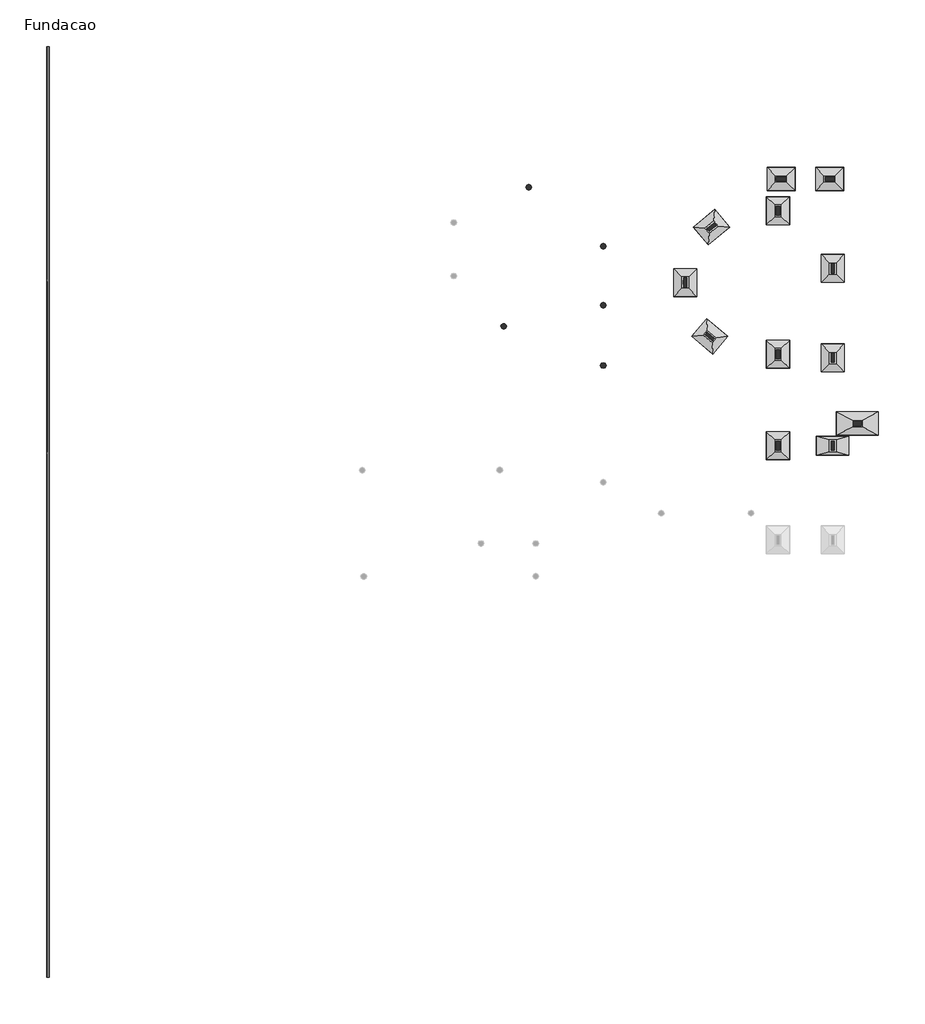
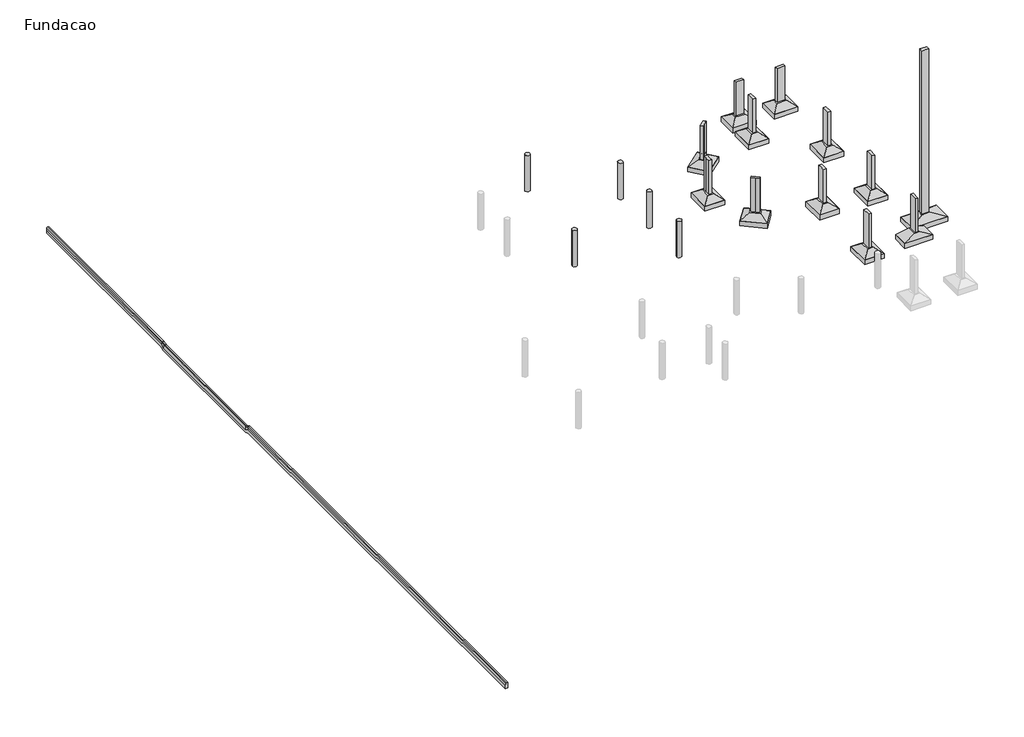
# One storey, part 2 of 2: 17 columns, 12 fasteners, 1 proxy.
# Revit data of these elements (continued)
# Element 4 (IfcColumn, "TQS - Pilar circular : TQS - Pilar circular 25.0cm") (continued)
#   Unir com o próximo = ""
#   Grupo pre moldado = ""
#   Verificado = ""
#   Concreto C = ""
#   Taxa de armadura (kgf/m³) = 0
#   Carga (tf/m²) = 0
#   Carga (tf/m) = 0
#   Carga (tf) = 0
#   Altura = 1.70 m
#   Rebaixo = 0.00 m
#   Altura da fundacao = 0.00 m
#   Largura = 0.00 m
#   Distancia a face = 0.00 m
#   Distancia ao eixo = 0.00 m
#   Resultado de Ensaios fck (MPa) = 0
#   Unique TQS ID = -767
#   Principal = yes
#   Nasce = yes
#   Morre = yes
#   Cabeca de Pilar = no
#   Structural Material = Concrete - Cast-in-Place Concrete
#   Phase Created = CC_AP/ESTR
#   Materials on its faces: "Concrete - Cast-in-Place Concrete"
# Element 5 (IfcColumn, "TQS - Pilar circular : TQS - Pilar circular 25.0cm")
#   Uso = "ESTRUTURA"
#   Titulo = "B3"
#   Chave = "B3//0"
#   Tipo Elemento = "Pilar"
#   SHA1 = "B4824BA6EB04DBA88013BAD919A11F987E93A8CE"
#   Revisão = ""
#   Tipo de carga = ""
#   Divisor de flexao = ""
#   Secao = "C 25"
#   Configuracao = ""
#   Angulo (graus) = ""
#   Detalhamento = ""
#   Casos de vento manual = ""
#   Tipo = ""
#   Alcas = ""
#   Furos = ""
#   Pino = ""
#   Distribuicao = ""
#   Solidarizado = ""
#   Solidarizar na montagem = ""
#   Unir com o próximo = ""
#   Grupo pre moldado = ""
#   Verificado = ""
#   Concreto C = ""
#   Taxa de armadura (kgf/m³) = 0
#   Carga (tf/m²) = 0
#   Carga (tf/m) = 0
#   Carga (tf) = 0
#   Altura = 1.70 m
#   Rebaixo = 0.00 m
#   Altura da fundacao = 0.00 m
#   Largura = 0.00 m
#   Distancia a face = 0.00 m
#   Distancia ao eixo = 0.00 m
#   Resultado de Ensaios fck (MPa) = 0
#   Unique TQS ID = -768
#   Principal = yes
#   Nasce = yes
#   Morre = yes
#   Cabeca de Pilar = no
#   Structural Material = Concrete - Cast-in-Place Concrete
#   Phase Created = CC_AP/ESTR
#   Materials on its faces: "Concrete - Cast-in-Place Concrete"
# Element 6 (IfcColumn, "TQS - Pilar circular : TQS - Pilar circular 25.0cm")
#   Uso = "ESTRUTURA"
#   Titulo = "B7"
#   Chave = "B7//0"
#   Tipo Elemento = "Pilar"
#   SHA1 = "0C09F8E52B5679DF636ED6AD079635606BCF1DE0"
#   Revisão = ""
#   Tipo de carga = ""
#   Divisor de flexao = ""
#   Secao = "C 25"
#   Configuracao = ""
#   Angulo (graus) = ""
#   Detalhamento = ""
#   Casos de vento manual = ""
#   Tipo = ""
#   Alcas = ""
#   Furos = ""
#   Pino = ""
#   Distribuicao = ""
#   Solidarizado = ""
#   Solidarizar na montagem = ""
#   Unir com o próximo = ""
#   Grupo pre moldado = ""
#   Verificado = ""
#   Concreto C = ""
#   Taxa de armadura (kgf/m³) = 0
#   Carga (tf/m²) = 0
#   Carga (tf/m) = 0
#   Carga (tf) = 0
#   Altura = 1.70 m
#   Rebaixo = 0.00 m
#   Altura da fundacao = 0.00 m
#   Largura = 0.00 m
#   Distancia a face = 0.00 m
#   Distancia ao eixo = 0.00 m
#   Resultado de Ensaios fck (MPa) = 0
#   Unique TQS ID = -769
#   Principal = yes
#   Nasce = yes
#   Morre = yes
#   Cabeca de Pilar = no
#   Structural Material = Concrete - Cast-in-Place Concrete
#   Phase Created = CC_AP/ESTR
#   Materials on its faces: "Concrete - Cast-in-Place Concrete"
# Element 7 (IfcColumn, "TQS - Pilar retangular : 14.0 x 40.0")
#   Uso = "ESTRUTURA"
#   Titulo = "PS1"
#   Chave = "PS1//0"
#   Tipo Elemento = "Pilar"
#   SHA1 = "4597F8CE5B5008DD3216867DEF2D1334C590FC15"
#   Revisão = ""
#   Tipo de carga = ""
#   Divisor de flexao = ""
#   Secao = "R 14/40 270°"
#   Configuracao = ""
#   Angulo (graus) = ""
#   Detalhamento = ""
#   Casos de vento manual = ""
#   Tipo = ""
#   Alcas = ""
#   Furos = ""
#   Pino = ""
#   Distribuicao = ""
#   Solidarizado = ""
#   Solidarizar na montagem = ""
#   Unir com o próximo = ""
#   Grupo pre moldado = ""
#   Verificado = ""
#   Concreto C = ""
#   Taxa de armadura (kgf/m³) = 0
#   Carga (tf/m²) = 0
#   Carga (tf/m) = 0
#   Carga (tf) = 0
#   Altura = 1.70 m
#   Rebaixo = 0.00 m
#   Altura da fundacao = 0.00 m
#   Largura = 0.00 m
#   Distancia a face = 0.00 m
#   Distancia ao eixo = 0.00 m
#   Resultado de Ensaios fck (MPa) = 0
#   Unique TQS ID = -958
#   Principal = yes
#   Nasce = yes
#   Morre = yes
#   Cabeca de Pilar = no
#   Structural Material = Concrete - Cast-in-Place Concrete
#   Phase Created = CC_AP/ESTR
#   Materials on its faces: "Concrete - Cast-in-Place Concrete"
# Element 8 (IfcColumn, "TQS - Pilar retangular : 14.0 x 40.0")
#   Uso = "ESTRUTURA"
#   Titulo = "PS2"
#   Chave = "PS2//0"
#   Tipo Elemento = "Pilar"
#   SHA1 = "1729CD9DA72122FACD843418D908847D3B1966CD"
#   Revisão = ""
#   Tipo de carga = ""
#   Divisor de flexao = ""
#   Secao = "R 14/40 270°"
#   Configuracao = ""
#   Angulo (graus) = ""
#   Detalhamento = ""
#   Casos de vento manual = ""
#   Tipo = ""
#   Alcas = ""
#   Furos = ""
#   Pino = ""
#   Distribuicao = ""
#   Solidarizado = ""
#   Solidarizar na montagem = ""
#   Unir com o próximo = ""
#   Grupo pre moldado = ""
#   Verificado = ""
#   Concreto C = ""
#   Taxa de armadura (kgf/m³) = 0
#   Carga (tf/m²) = 0
#   Carga (tf/m) = 0
#   Carga (tf) = 0
#   Altura = 1.70 m
#   Rebaixo = 0.00 m
#   Altura da fundacao = 0.00 m
#   Largura = 0.00 m
#   Distancia a face = 0.00 m
#   Distancia ao eixo = 0.00 m
#   Resultado de Ensaios fck (MPa) = 0
#   Unique TQS ID = -959
#   Principal = yes
#   Nasce = yes
#   Morre = yes
#   Cabeca de Pilar = no
#   Structural Material = Concrete - Cast-in-Place Concrete
#   Phase Created = CC_AP/ESTR
#   Materials on its faces: "Concrete - Cast-in-Place Concrete"
# Element 9 (IfcColumn, "TQS - Pilar retangular : 14.0 x 40.0")
#   Uso = "ESTRUTURA"
#   Titulo = "PS3"
#   Chave = "PS3//0"
#   Tipo Elemento = "Pilar"
#   SHA1 = "E1C4E1DD2B85E2F78CE9D8770BC24705A0EC4463"
#   Revisão = ""
#   Tipo de carga = ""
#   Divisor de flexao = ""
#   Secao = "R 14/40 180°"
#   Configuracao = ""
#   Angulo (graus) = ""
#   Detalhamento = ""
#   Casos de vento manual = ""
#   Tipo = ""
#   Alcas = ""
#   Furos = ""
#   Pino = ""
#   Distribuicao = ""
#   Solidarizado = ""
#   Solidarizar na montagem = ""
#   Unir com o próximo = ""
#   Grupo pre moldado = ""
#   Verificado = ""
#   Concreto C = ""
#   Taxa de armadura (kgf/m³) = 0
#   Carga (tf/m²) = 0
#   Carga (tf/m) = 0
#   Carga (tf) = 0
#   Altura = 1.70 m
#   Rebaixo = 0.00 m
#   Altura da fundacao = 0.00 m
#   Largura = 0.00 m
#   Distancia a face = 0.00 m
#   Distancia ao eixo = 0.00 m
#   Resultado de Ensaios fck (MPa) = 0
#   Unique TQS ID = -960
#   Principal = yes
#   Nasce = yes
#   Morre = yes
#   Cabeca de Pilar = no
#   Structural Material = Concrete - Cast-in-Place Concrete
#   Phase Created = CC_AP/ESTR
#   Materials on its faces: "Concrete - Cast-in-Place Concrete"
# Element 10 (IfcColumn, "TQS - Pilar retangular : 14.0 x 40.0")
#   Uso = "ESTRUTURA"
#   Titulo = "PS7"
#   Chave = "PS7//0"
#   Tipo Elemento = "Pilar"
#   SHA1 = "EE51B7F018C373FE9CEF53A9864C8051348A9FB9"
#   Revisão = ""
#   Tipo de carga = ""
#   Divisor de flexao = ""
#   Secao = "R 14/40 180°"
#   Configuracao = ""
#   Angulo (graus) = ""
#   Detalhamento = ""
#   Casos de vento manual = ""
#   Tipo = ""
#   Alcas = ""
#   Furos = ""
#   Pino = ""
#   Distribuicao = ""
#   Solidarizado = ""
#   Solidarizar na montagem = ""
#   Unir com o próximo = ""
#   Grupo pre moldado = ""
#   Verificado = ""
#   Concreto C = ""
#   Taxa de armadura (kgf/m³) = 0
#   Carga (tf/m²) = 0
#   Carga (tf/m) = 0
#   Carga (tf) = 0
#   Altura = 1.70 m
#   Rebaixo = 0.00 m
#   Altura da fundacao = 0.00 m
#   Largura = 0.00 m
#   Distancia a face = 0.00 m
#   Distancia ao eixo = 0.00 m
#   Resultado de Ensaios fck (MPa) = 0
#   Unique TQS ID = -964
#   Principal = yes
#   Nasce = yes
#   Morre = yes
#   Cabeca de Pilar = no
#   Structural Material = Concrete - Cast-in-Place Concrete
#   Phase Created = CC_AP/ESTR
#   Materials on its faces: "Concrete - Cast-in-Place Concrete"
# Element 11 (IfcColumn, "TQS - Pilar retangular : 14.0 x 40.0")
#   Uso = "ESTRUTURA"
#   Titulo = "PS8"
#   Chave = "PS8//0"
#   Tipo Elemento = "Pilar"
#   SHA1 = "B515A8CC25CBD0A114828B82A1075E16319BC015"
#   Revisão = ""
#   Tipo de carga = ""
#   Divisor de flexao = ""
#   Secao = "R 14/40 180°"
#   Configuracao = ""
#   Angulo (graus) = ""
#   Detalhamento = ""
#   Casos de vento manual = ""
#   Tipo = ""
#   Alcas = ""
#   Furos = ""
#   Pino = ""
#   Distribuicao = ""
#   Solidarizado = ""
#   Solidarizar na montagem = ""
#   Unir com o próximo = ""
#   Grupo pre moldado = ""
#   Verificado = ""
#   Concreto C = ""
#   Taxa de armadura (kgf/m³) = 0
#   Carga (tf/m²) = 0
#   Carga (tf/m) = 0
#   Carga (tf) = 0
#   Altura = 1.70 m
#   Rebaixo = 0.00 m
#   Altura da fundacao = 0.00 m
#   Largura = 0.00 m
#   Distancia a face = 0.00 m
#   Distancia ao eixo = 0.00 m
#   Resultado de Ensaios fck (MPa) = 0
#   Unique TQS ID = -965
#   Principal = yes
#   Nasce = yes
#   Morre = yes
#   Cabeca de Pilar = no
#   Structural Material = Concrete - Cast-in-Place Concrete
#   Phase Created = CC_AP/ESTR
#   Materials on its faces: "Concrete - Cast-in-Place Concrete"
# Element 12 (IfcColumn, "TQS - Pilar retangular : 14.0 x 40.0")
#   Uso = "ESTRUTURA"
#   Titulo = "PS11"
#   Chave = "PS11//0"
#   Tipo Elemento = "Pilar"
#   SHA1 = "38C3E9E25C80C043D595FE86FE1A911FDC38D350"
#   Revisão = ""
#   Tipo de carga = ""
#   Divisor de flexao = ""
#   Secao = "R 14/40 180°"
#   Configuracao = ""
#   Angulo (graus) = ""
#   Detalhamento = ""
#   Casos de vento manual = ""
#   Tipo = ""
#   Alcas = ""
#   Furos = ""
#   Pino = ""
#   Distribuicao = ""
#   Solidarizado = ""
#   Solidarizar na montagem = ""
#   Unir com o próximo = ""
#   Grupo pre moldado = ""
#   Verificado = ""
#   Concreto C = ""
#   Taxa de armadura (kgf/m³) = 0
#   Carga (tf/m²) = 0
#   Carga (tf/m) = 0
#   Carga (tf) = 0
#   Altura = 1.70 m
#   Rebaixo = 0.00 m
#   Altura da fundacao = 0.00 m
#   Largura = 0.00 m
#   Distancia a face = 0.00 m
#   Distancia ao eixo = 0.00 m
#   Resultado de Ensaios fck (MPa) = 0
#   Unique TQS ID = -968
#   Principal = yes
#   Nasce = yes
#   Morre = yes
#   Cabeca de Pilar = no
#   Structural Material = Concrete - Cast-in-Place Concrete
#   Phase Created = CC_AP/ESTR
#   Materials on its faces: "Concrete - Cast-in-Place Concrete"
# Element 13 (IfcColumn, "TQS - Pilar retangular : 14.0 x 40.0")
#   Uso = "ESTRUTURA"
#   Titulo = "PS12"
#   Chave = "PS12//0"
#   Tipo Elemento = "Pilar"
#   SHA1 = "512D0DE7DB718BC0FE0AECE12A9FB23F7FBE26A9"
#   Revisão = ""
#   Tipo de carga = ""
#   Divisor de flexao = ""
#   Secao = "R 14/40 180°"
#   Configuracao = ""
#   Angulo (graus) = ""
#   Detalhamento = ""
#   Casos de vento manual = ""
#   Tipo = ""
#   Alcas = ""
#   Furos = ""
#   Pino = ""
#   Distribuicao = ""
#   Solidarizado = ""
#   Solidarizar na montagem = ""
#   Unir com o próximo = ""
#   Grupo pre moldado = ""
#   Verificado = ""
#   Concreto C = ""
#   Taxa de armadura (kgf/m³) = 0
#   Carga (tf/m²) = 0
#   Carga (tf/m) = 0
#   Carga (tf) = 0
#   Altura = 1.70 m
#   Rebaixo = 0.00 m
#   Altura da fundacao = 0.00 m
#   Largura = 0.00 m
#   Distancia a face = 0.00 m
#   Distancia ao eixo = 0.00 m
#   Resultado de Ensaios fck (MPa) = 0
#   Unique TQS ID = -969
#   Principal = yes
#   Nasce = yes
#   Morre = yes
#   Cabeca de Pilar = no
#   Structural Material = Concrete - Cast-in-Place Concrete
#   Phase Created = CC_AP/ESTR
#   Materials on its faces: "Concrete - Cast-in-Place Concrete"
# Element 14 (IfcColumn, "TQS - Pilar retangular : 14.0 x 40.0")
#   Uso = "ESTRUTURA"
#   Titulo = "PS13"
#   Chave = "PS13//0"
#   Tipo Elemento = "Pilar"
#   SHA1 = "8EC8E2C6B90DD4DF760F1D4ED431316ED84D10F2"
#   Revisão = ""
#   Tipo de carga = ""
#   Divisor de flexao = ""
#   Secao = "R 14/40 180°"
#   Configuracao = ""
#   Angulo (graus) = ""
#   Detalhamento = ""
#   Casos de vento manual = ""
#   Tipo = ""
#   Alcas = ""
#   Furos = ""
#   Pino = ""
#   Distribuicao = ""
#   Solidarizado = ""
#   Solidarizar na montagem = ""
#   Unir com o próximo = ""
#   Grupo pre moldado = ""
#   Verificado = ""
#   Concreto C = ""
#   Taxa de armadura (kgf/m³) = 0
#   Carga (tf/m²) = 0
#   Carga (tf/m) = 0
#   Carga (tf) = 0
#   Altura = 1.70 m
#   Rebaixo = 0.00 m
#   Altura da fundacao = 0.00 m
#   Largura = 0.00 m
#   Distancia a face = 0.00 m
#   Distancia ao eixo = 0.00 m
#   Resultado de Ensaios fck (MPa) = 0
#   Unique TQS ID = -970
#   Principal = yes
#   Nasce = yes
#   Morre = yes
#   Cabeca de Pilar = no
#   Structural Material = Concrete - Cast-in-Place Concrete
#   Phase Created = CC_AP/ESTR
#   Materials on its faces: "Concrete - Cast-in-Place Concrete"
# Element 15 (IfcColumn, "TQS - Pilar retangular : 19.0 x 35.0")
#   Uso = "ESTRUTURA"
#   Titulo = "P14"
#   Chave = "P14//0"
#   Tipo Elemento = "Pilar"
#   SHA1 = "6631C03D899D7914EBA5EACF44BE1498A45C603B"
#   Revisão = ""
#   Tipo de carga = ""
#   Divisor de flexao = ""
#   Secao = "R 19/35 90°"
#   Configuracao = ""
#   Angulo (graus) = ""
#   Detalhamento = ""
#   Casos de vento manual = ""
#   Tipo = ""
#   Alcas = ""
#   Furos = ""
#   Pino = ""
#   Distribuicao = ""
#   Solidarizado = ""
#   Solidarizar na montagem = ""
#   Unir com o próximo = ""
#   Grupo pre moldado = ""
#   Verificado = ""
#   Concreto C = ""
#   Taxa de armadura (kgf/m³) = 0
#   Carga (tf/m²) = 0
#   Carga (tf/m) = 0
#   Carga (tf) = 0
#   Altura = 7.85 m
#   Rebaixo = 0.00 m
#   Altura da fundacao = 0.00 m
#   Largura = 0.00 m
#   Distancia a face = 0.00 m
#   Distancia ao eixo = 0.00 m
#   Resultado de Ensaios fck (MPa) = 0
#   Unique TQS ID = -30
#   Principal = yes
#   Nasce = yes
#   Morre = yes
#   Cabeca de Pilar = no
#   Structural Material = Concrete - Cast-in-Place Concrete
#   Phase Created = CC_AP/ESTR
#   Materials on its faces: "Concrete - Cast-in-Place Concrete"
# Element 16 (IfcColumn, "TQS - Pilar Polig_1 : TQS Column")
#   Uso = "ESTRUTURA"
#   Titulo = "PS4"
#   Chave = "PS4//0"
#   Tipo Elemento = "Pilar"
#   SHA1 = "CAF5758E71A5FE097847EBD6542E0EE23CE53B7B"
#   Revisão = ""
#   Tipo de carga = ""
#   Divisor de flexao = ""
#   Secao = "P  - Poligonal"
#   Configuracao = ""
#   Angulo (graus) = ""
#   Detalhamento = ""
#   Casos de vento manual = ""
#   Tipo = ""
#   Alcas = ""
#   Furos = ""
#   Pino = ""
#   Distribuicao = ""
#   Solidarizado = ""
#   Solidarizar na montagem = ""
#   Unir com o próximo = ""
#   Grupo pre moldado = ""
#   Verificado = ""
#   Concreto C = ""
#   Taxa de armadura (kgf/m³) = 0
#   Carga (tf/m²) = 0
#   Carga (tf/m) = 0
#   Carga (tf) = 0
#   Altura = 1.70 m
#   Rebaixo = 0.00 m
#   Altura da fundacao = 0.00 m
#   Largura = 0.00 m
#   Distancia a face = 0.00 m
#   Distancia ao eixo = 0.00 m
#   Resultado de Ensaios fck (MPa) = 0
#   Unique TQS ID = -961
#   Principal = yes
#   Nasce = yes
#   Morre = yes
#   Cabeca de Pilar = no
#   Structural Material = Concrete - Cast-in-Place Concrete
#   Phase Created = CC_AP/ESTR
# Element 17 (IfcColumn, "TQS - Pilar Polig_1 : TQS Column")
#   Uso = "ESTRUTURA"
#   Titulo = "PS5"
#   Chave = "PS5//0"
#   Tipo Elemento = "Pilar"
#   SHA1 = "AE9BDBDC0B1786B9555B7E0CE4AAD4E849800AD1"
#   Revisão = ""
#   Tipo de carga = ""
#   Divisor de flexao = ""
#   Secao = "P  - Poligonal"
#   Configuracao = ""
#   Angulo (graus) = ""
#   Detalhamento = ""
#   Casos de vento manual = ""
#   Tipo = ""
#   Alcas = ""
#   Furos = ""
#   Pino = ""
#   Distribuicao = ""
#   Solidarizado = ""
#   Solidarizar na montagem = ""
#   Unir com o próximo = ""
#   Grupo pre moldado = ""
#   Verificado = ""
#   Concreto C = ""
#   Taxa de armadura (kgf/m³) = 0
#   Carga (tf/m²) = 0
#   Carga (tf/m) = 0
#   Carga (tf) = 0
#   Altura = 1.70 m
#   Rebaixo = 0.00 m
#   Altura da fundacao = 0.00 m
#   Largura = 0.00 m
#   Distancia a face = 0.00 m
#   Distancia ao eixo = 0.00 m
#   Resultado de Ensaios fck (MPa) = 0
#   Unique TQS ID = -962
#   Principal = yes
#   Nasce = yes
#   Morre = yes
#   Cabeca de Pilar = no
#   Structural Material = Concrete - Cast-in-Place Concrete
#   Phase Created = CC_AP/ESTR
# Element 18 (IfcColumn, "TQS - Pilar Polig_2 : TQS Column")
#   Uso = "ESTRUTURA"
#   Titulo = "PS6"
#   Chave = "PS6//0"
#   Tipo Elemento = "Pilar"
#   SHA1 = "07EEAEB0E5A3D9C7C5812BCB6FDA506A68E4D4F2"
#   Revisão = ""
#   Tipo de carga = ""
#   Divisor de flexao = ""
#   Secao = "P  - Poligonal"
#   Configuracao = ""
#   Angulo (graus) = ""
#   Detalhamento = ""
#   Casos de vento manual = ""
#   Tipo = ""
#   Alcas = ""
#   Furos = ""
#   Pino = ""
#   Distribuicao = ""
#   Solidarizado = ""
#   Solidarizar na montagem = ""
#   Unir com o próximo = ""
#   Grupo pre moldado = ""
#   Verificado = ""
#   Concreto C = ""
#   Taxa de armadura (kgf/m³) = 0
#   Carga (tf/m²) = 0
#   Carga (tf/m) = 0
#   Carga (tf) = 0
#   Altura = 1.70 m
#   Rebaixo = 0.00 m
#   Altura da fundacao = 0.00 m
#   Largura = 0.00 m
#   Distancia a face = 0.00 m
#   Distancia ao eixo = 0.00 m
#   Resultado de Ensaios fck (MPa) = 0
#   Unique TQS ID = -963
#   Principal = yes
#   Nasce = yes
#   Morre = yes
#   Cabeca de Pilar = no
#   Structural Material = Concrete - Cast-in-Place Concrete
#   Phase Created = CC_AP/ESTR
# Element 19 (IfcFastener, "TQS - Sapata : S14")
#   Uso = "ESTRUTURA"
#   Titulo = "S14"
#   Chave = "-1550"
#   Tipo Elemento = "Fundação"
#   SHA1 = "1357E856F80250D7EFC9EC1E050D5963CC884844"
#   Revisão = ""
#   Tipo de carga = ""
#   Divisor de flexao = ""
#   Secao = ""
#   Configuracao = ""
#   Angulo (graus) = ""
#   Detalhamento = ""
#   Casos de vento manual = ""
#   Tipo = "Sapata"
#   Dimensoes = "100.0,180.0"
#   Estacas = ""
#   Calice = ""
#   Rugosidade = ""
#   Alcas = ""
#   Furos = ""
#   Pino = ""
#   Distribuicao = ""
#   Solidarizado = ""
#   Solidarizar na montagem = ""
#   Unir com o próximo = ""
#   Grupo pre moldado = ""
#   Verificado = ""
#   Concreto C = ""
#   Taxa de armadura (kgf/m³) = 0
#   Carga (tf/m²) = 0
#   Carga (tf/m) = 0
#   Carga (tf) = 0
#   Altura = 0.00 m
#   Rebaixo = 0.00 m
#   Pilar ficticio = 0.00 m
#   Topo = -1.45 m
#   Altura total = 0.50 m
#   Rodape = 0.00 m
#   Diametro = 0.00 m
#   Altura dentro do bloco = 0.00 m
#   Entre eixos = 0.00 m
#   Paredes = 0.00 m
#   Caimento = 0.00 m
#   Largura = 0.00 m
#   Distancia a face = 0.00 m
#   Distancia ao eixo = 0.00 m
#   Resultado de Ensaios fck (MPa) = 0
#   Unique TQS ID = -1550
#   Principal = yes
#   Phase Created = CC_AP/ESTR
#   Materials on its faces: "Concreto - Concreto concretado no local"
# Element 20 (IfcFastener, "TQS - Sapata : SPS1")
#   Uso = "ESTRUTURA"
#   Titulo = "SPS1"
#   Chave = "-1512"
#   Tipo Elemento = "Fundação"
#   SHA1 = "0DB0C78ACFE2E409544A77F7853F60381CB93818"
#   Revisão = ""
#   Tipo de carga = ""
#   Divisor de flexao = ""
#   Secao = ""
#   Configuracao = ""
#   Angulo (graus) = ""
#   Detalhamento = ""
#   Casos de vento manual = ""
#   Tipo = "Sapata"
#   Dimensoes = "100.0,120.0"
#   Estacas = ""
#   Calice = ""
#   Rugosidade = ""
#   Alcas = ""
#   Furos = ""
#   Pino = ""
#   Distribuicao = ""
#   Solidarizado = ""
#   Solidarizar na montagem = ""
#   Unir com o próximo = ""
#   Grupo pre moldado = ""
#   Verificado = ""
#   Concreto C = ""
#   Taxa de armadura (kgf/m³) = 0
#   Carga (tf/m²) = 0
#   Carga (tf/m) = 0
#   Carga (tf) = 0
#   Altura = 0.00 m
#   Rebaixo = 0.00 m
#   Pilar ficticio = 0.00 m
#   Topo = -1.45 m
#   Altura total = 0.50 m
#   Rodape = 0.00 m
#   Diametro = 0.00 m
#   Altura dentro do bloco = 0.00 m
#   Entre eixos = 0.00 m
#   Paredes = 0.00 m
#   Caimento = 0.00 m
#   Largura = 0.00 m
#   Distancia a face = 0.00 m
#   Distancia ao eixo = 0.00 m
#   Resultado de Ensaios fck (MPa) = 0
#   Unique TQS ID = -1512
#   Principal = yes
#   Phase Created = CC_AP/ESTR
#   Materials on its faces: "Concreto - Concreto concretado no local"
# Element 21 (IfcFastener, "TQS - Sapata : SPS11")
#   Uso = "ESTRUTURA"
#   Titulo = "SPS11"
#   Chave = "-1544"
#   Tipo Elemento = "Fundação"
#   SHA1 = "678A094029D3186700C53CC9859E21CCB03EEAB8"
#   Revisão = ""
#   Tipo de carga = ""
#   Divisor de flexao = ""
#   Secao = ""
#   Configuracao = ""
#   Angulo (graus) = ""
#   Detalhamento = ""
#   Casos de vento manual = ""
#   Tipo = "Sapata"
#   Dimensoes = "140.0,80.0"
#   Estacas = ""
#   Calice = ""
#   Rugosidade = ""
#   Alcas = ""
#   Furos = ""
#   Pino = ""
#   Distribuicao = ""
#   Solidarizado = ""
#   Solidarizar na montagem = ""
#   Unir com o próximo = ""
#   Grupo pre moldado = ""
#   Verificado = ""
#   Concreto C = ""
#   Taxa de armadura (kgf/m³) = 0
#   Carga (tf/m²) = 0
#   Carga (tf/m) = 0
#   Carga (tf) = 0
#   Altura = 0.00 m
#   Rebaixo = 0.00 m
#   Pilar ficticio = 0.00 m
#   Topo = -1.45 m
#   Altura total = 0.50 m
#   Rodape = 0.00 m
#   Diametro = 0.00 m
#   Altura dentro do bloco = 0.00 m
#   Entre eixos = 0.00 m
#   Paredes = 0.00 m
#   Caimento = 0.00 m
#   Largura = 0.00 m
#   Distancia a face = 0.00 m
#   Distancia ao eixo = 0.00 m
#   Resultado de Ensaios fck (MPa) = 0
#   Unique TQS ID = -1544
#   Principal = yes
#   Phase Created = CC_AP/ESTR
#   Materials on its faces: "Concreto - Concreto concretado no local"
# Element 22 (IfcFastener, "TQS - Sapata : SPS12")
#   Uso = "ESTRUTURA"
#   Titulo = "SPS12"
#   Chave = "-1545"
#   Tipo Elemento = "Fundação"
#   SHA1 = "A892B9C9285BE3407F8B32028442AB264075CE3A"
#   Revisão = ""
#   Tipo de carga = ""
#   Divisor de flexao = ""
#   Secao = ""
#   Configuracao = ""
#   Angulo (graus) = ""
#   Detalhamento = ""
#   Casos de vento manual = ""
#   Tipo = "Sapata"
#   Dimensoes = "100.0,120.0"
#   Estacas = ""
#   Calice = ""
#   Rugosidade = ""
#   Alcas = ""
#   Furos = ""
#   Pino = ""
#   Distribuicao = ""
#   Solidarizado = ""
#   Solidarizar na montagem = ""
#   Unir com o próximo = ""
#   Grupo pre moldado = ""
#   Verificado = ""
#   Concreto C = ""
#   Taxa de armadura (kgf/m³) = 0
#   Carga (tf/m²) = 0
#   Carga (tf/m) = 0
#   Carga (tf) = 0
#   Altura = 0.00 m
#   Rebaixo = 0.00 m
#   Pilar ficticio = 0.00 m
#   Topo = -1.45 m
#   Altura total = 0.50 m
#   Rodape = 0.00 m
#   Diametro = 0.00 m
#   Altura dentro do bloco = 0.00 m
#   Entre eixos = 0.00 m
#   Paredes = 0.00 m
#   Caimento = 0.00 m
#   Largura = 0.00 m
#   Distancia a face = 0.00 m
#   Distancia ao eixo = 0.00 m
#   Resultado de Ensaios fck (MPa) = 0
#   Unique TQS ID = -1545
#   Principal = yes
#   Phase Created = CC_AP/ESTR
#   Materials on its faces: "Concreto - Concreto concretado no local"
# Element 23 (IfcFastener, "TQS - Sapata : SPS13")
#   Uso = "ESTRUTURA"
#   Titulo = "SPS13"
#   Chave = "-1546"
#   Tipo Elemento = "Fundação"
#   SHA1 = "CDD7149D511DCC0D87C76189E976442BBC013FA0"
#   Revisão = ""
#   Tipo de carga = ""
#   Divisor de flexao = ""
#   Secao = ""
#   Configuracao = ""
#   Angulo (graus) = ""
#   Detalhamento = ""
#   Casos de vento manual = ""
#   Tipo = "Sapata"
#   Dimensoes = "100.0,120.0"
#   Estacas = ""
#   Calice = ""
#   Rugosidade = ""
#   Alcas = ""
#   Furos = ""
#   Pino = ""
#   Distribuicao = ""
#   Solidarizado = ""
#   Solidarizar na montagem = ""
#   Unir com o próximo = ""
#   Grupo pre moldado = ""
#   Verificado = ""
#   Concreto C = ""
#   Taxa de armadura (kgf/m³) = 0
#   Carga (tf/m²) = 0
#   Carga (tf/m) = 0
#   Carga (tf) = 0
#   Altura = 0.00 m
#   Rebaixo = 0.00 m
#   Pilar ficticio = 0.00 m
#   Topo = -1.45 m
#   Altura total = 0.50 m
#   Rodape = 0.00 m
#   Diametro = 0.00 m
#   Altura dentro do bloco = 0.00 m
#   Entre eixos = 0.00 m
#   Paredes = 0.00 m
#   Caimento = 0.00 m
#   Largura = 0.00 m
#   Distancia a face = 0.00 m
#   Distancia ao eixo = 0.00 m
#   Resultado de Ensaios fck (MPa) = 0
#   Unique TQS ID = -1546
#   Principal = yes
#   Phase Created = CC_AP/ESTR
#   Materials on its faces: "Concreto - Concreto concretado no local"
# Element 24 (IfcFastener, "TQS - Sapata : SPS2")
#   Uso = "ESTRUTURA"
#   Titulo = "SPS2"
#   Chave = "-1513"
#   Tipo Elemento = "Fundação"
#   SHA1 = "603FADD6DB2EB68781E32AEC81705DC053729A4E"
#   Revisão = ""
#   Tipo de carga = ""
#   Divisor de flexao = ""
#   Secao = ""
#   Configuracao = ""
#   Angulo (graus) = ""
#   Detalhamento = ""
#   Casos de vento manual = ""
#   Tipo = "Sapata"
#   Dimensoes = "100.0,120.0"
#   Estacas = ""
#   Calice = ""
#   Rugosidade = ""
#   Alcas = ""
#   Furos = ""
#   Pino = ""
#   Distribuicao = ""
#   Solidarizado = ""
#   Solidarizar na montagem = ""
#   Unir com o próximo = ""
#   Grupo pre moldado = ""
#   Verificado = ""
#   Concreto C = ""
#   Taxa de armadura (kgf/m³) = 0
#   Carga (tf/m²) = 0
#   Carga (tf/m) = 0
#   Carga (tf) = 0
#   Altura = 0.00 m
#   Rebaixo = 0.00 m
#   Pilar ficticio = 0.00 m
#   Topo = -1.45 m
#   Altura total = 0.50 m
#   Rodape = 0.00 m
#   Diametro = 0.00 m
#   Altura dentro do bloco = 0.00 m
#   Entre eixos = 0.00 m
#   Paredes = 0.00 m
#   Caimento = 0.00 m
#   Largura = 0.00 m
#   Distancia a face = 0.00 m
#   Distancia ao eixo = 0.00 m
#   Resultado de Ensaios fck (MPa) = 0
#   Unique TQS ID = -1513
#   Principal = yes
#   Phase Created = CC_AP/ESTR
#   Materials on its faces: "Concreto - Concreto concretado no local"
# Element 25 (IfcFastener, "TQS - Sapata : SPS3")
#   Uso = "ESTRUTURA"
#   Titulo = "SPS3"
#   Chave = "-1536"
#   Tipo Elemento = "Fundação"
#   SHA1 = "79306587FBF9E385D4E688BE4182F1340258C694"
#   Revisão = ""
#   Tipo de carga = ""
#   Divisor de flexao = ""
#   Secao = ""
#   Configuracao = ""
#   Angulo (graus) = ""
#   Detalhamento = ""
#   Casos de vento manual = ""
#   Tipo = "Sapata"
#   Dimensoes = "100.0,120.0"
#   Estacas = ""
#   Calice = ""
#   Rugosidade = ""
#   Alcas = ""
#   Furos = ""
#   Pino = ""
#   Distribuicao = ""
#   Solidarizado = ""
#   Solidarizar na montagem = ""
#   Unir com o próximo = ""
#   Grupo pre moldado = ""
#   Verificado = ""
#   Concreto C = ""
#   Taxa de armadura (kgf/m³) = 0
#   Carga (tf/m²) = 0
#   Carga (tf/m) = 0
#   Carga (tf) = 0
#   Altura = 0.00 m
#   Rebaixo = 0.00 m
#   Pilar ficticio = 0.00 m
#   Topo = -1.45 m
#   Altura total = 0.50 m
#   Rodape = 0.00 m
#   Diametro = 0.00 m
#   Altura dentro do bloco = 0.00 m
#   Entre eixos = 0.00 m
#   Paredes = 0.00 m
#   Caimento = 0.00 m
#   Largura = 0.00 m
#   Distancia a face = 0.00 m
#   Distancia ao eixo = 0.00 m
#   Resultado de Ensaios fck (MPa) = 0
#   Unique TQS ID = -1536
#   Principal = yes
#   Phase Created = CC_AP/ESTR
#   Materials on its faces: "Concreto - Concreto concretado no local"
# Element 26 (IfcFastener, "TQS - Sapata : SPS4")
#   Uso = "ESTRUTURA"
#   Titulo = "SPS4"
#   Chave = "-1537"
#   Tipo Elemento = "Fundação"
#   SHA1 = "C7F246035C6D677E4D229288FD6DAFF5BD781782"
#   Revisão = ""
#   Tipo de carga = ""
#   Divisor de flexao = ""
#   Secao = ""
#   Configuracao = ""
#   Angulo (graus) = ""
#   Detalhamento = ""
#   Casos de vento manual = ""
#   Tipo = "Sapata"
#   Dimensoes = "100.0,120.0"
#   Estacas = ""
#   Calice = ""
#   Rugosidade = ""
#   Alcas = ""
#   Furos = ""
#   Pino = ""
#   Distribuicao = ""
#   Solidarizado = ""
#   Solidarizar na montagem = ""
#   Unir com o próximo = ""
#   Grupo pre moldado = ""
#   Verificado = ""
#   Concreto C = ""
#   Taxa de armadura (kgf/m³) = 0
#   Carga (tf/m²) = 0
#   Carga (tf/m) = 0
#   Carga (tf) = 0
#   Altura = 0.00 m
#   Rebaixo = 0.00 m
#   Pilar ficticio = 0.00 m
#   Topo = -1.45 m
#   Altura total = 0.50 m
#   Rodape = 0.00 m
#   Diametro = 0.00 m
#   Altura dentro do bloco = 0.00 m
#   Entre eixos = 0.00 m
#   Paredes = 0.00 m
#   Caimento = 0.00 m
#   Largura = 0.00 m
#   Distancia a face = 0.00 m
#   Distancia ao eixo = 0.00 m
#   Resultado de Ensaios fck (MPa) = 0
#   Unique TQS ID = -1537
#   Principal = yes
#   Phase Created = CC_AP/ESTR
#   Materials on its faces: "Concreto - Concreto concretado no local"
# Element 27 (IfcFastener, "TQS - Sapata : SPS5")
#   Uso = "ESTRUTURA"
#   Titulo = "SPS5"
#   Chave = "-1538"
#   Tipo Elemento = "Fundação"
#   SHA1 = "42CB63A1D6FD1F93305BB9397719DE24CD6D6A3F"
#   Revisão = ""
#   Tipo de carga = ""
#   Divisor de flexao = ""
#   Secao = ""
#   Configuracao = ""
#   Angulo (graus) = ""
#   Detalhamento = ""
#   Casos de vento manual = ""
#   Tipo = "Sapata"
#   Dimensoes = "100.0,120.0"
#   Estacas = ""
#   Calice = ""
#   Rugosidade = ""
#   Alcas = ""
#   Furos = ""
#   Pino = ""
#   Distribuicao = ""
#   Solidarizado = ""
#   Solidarizar na montagem = ""
#   Unir com o próximo = ""
#   Grupo pre moldado = ""
#   Verificado = ""
#   Concreto C = ""
#   Taxa de armadura (kgf/m³) = 0
#   Carga (tf/m²) = 0
#   Carga (tf/m) = 0
#   Carga (tf) = 0
#   Altura = 0.00 m
#   Rebaixo = 0.00 m
#   Pilar ficticio = 0.00 m
#   Topo = -1.45 m
#   Altura total = 0.50 m
#   Rodape = 0.00 m
#   Diametro = 0.00 m
#   Altura dentro do bloco = 0.00 m
#   Entre eixos = 0.00 m
#   Paredes = 0.00 m
#   Caimento = 0.00 m
#   Largura = 0.00 m
#   Distancia a face = 0.00 m
#   Distancia ao eixo = 0.00 m
#   Resultado de Ensaios fck (MPa) = 0
#   Unique TQS ID = -1538
#   Principal = yes
#   Phase Created = CC_AP/ESTR
#   Materials on its faces: "Concreto - Concreto concretado no local"
# Element 28 (IfcFastener, "TQS - Sapata : SPS6")
#   Uso = "ESTRUTURA"
#   Titulo = "SPS6"
#   Chave = "-1539"
#   Tipo Elemento = "Fundação"
#   SHA1 = "7089DE54C758E879502D9964BA83D8ECE2A73D29"
#   Revisão = ""
#   Tipo de carga = ""
#   Divisor de flexao = ""
#   Secao = ""
#   Configuracao = ""
#   Angulo (graus) = ""
#   Detalhamento = ""
#   Casos de vento manual = ""
#   Tipo = "Sapata"
#   Dimensoes = "100.0,120.0"
#   Estacas = ""
#   Calice = ""
#   Rugosidade = ""
#   Alcas = ""
#   Furos = ""
#   Pino = ""
#   Distribuicao = ""
#   Solidarizado = ""
#   Solidarizar na montagem = ""
#   Unir com o próximo = ""
#   Grupo pre moldado = ""
#   Verificado = ""
#   Concreto C = ""
#   Taxa de armadura (kgf/m³) = 0
#   Carga (tf/m²) = 0
#   Carga (tf/m) = 0
#   Carga (tf) = 0
#   Altura = 0.00 m
#   Rebaixo = 0.00 m
#   Pilar ficticio = 0.00 m
#   Topo = -1.45 m
#   Altura total = 0.50 m
#   Rodape = 0.00 m
#   Diametro = 0.00 m
#   Altura dentro do bloco = 0.00 m
#   Entre eixos = 0.00 m
#   Paredes = 0.00 m
#   Caimento = 0.00 m
#   Largura = 0.00 m
#   Distancia a face = 0.00 m
#   Distancia ao eixo = 0.00 m
#   Resultado de Ensaios fck (MPa) = 0
#   Unique TQS ID = -1539
#   Principal = yes
#   Phase Created = CC_AP/ESTR
#   Materials on its faces: "Concreto - Concreto concretado no local"
# Element 29 (IfcFastener, "TQS - Sapata : SPS7")
#   Uso = "ESTRUTURA"
#   Titulo = "SPS7"
#   Chave = "-1540"
#   Tipo Elemento = "Fundação"
#   SHA1 = "39B73FB21C78E38761EEBB9B530BC320EF12A224"
#   Revisão = ""
#   Tipo de carga = ""
#   Divisor de flexao = ""
#   Secao = ""
#   Configuracao = ""
#   Angulo (graus) = ""
#   Detalhamento = ""
#   Casos de vento manual = ""
#   Tipo = "Sapata"
#   Dimensoes = "100.0,120.0"
#   Estacas = ""
#   Calice = ""
#   Rugosidade = ""
#   Alcas = ""
#   Furos = ""
#   Pino = ""
#   Distribuicao = ""
#   Solidarizado = ""
#   Solidarizar na montagem = ""
#   Unir com o próximo = ""
#   Grupo pre moldado = ""
#   Verificado = ""
#   Concreto C = ""
#   Taxa de armadura (kgf/m³) = 0
#   Carga (tf/m²) = 0
#   Carga (tf/m) = 0
#   Carga (tf) = 0
#   Altura = 0.00 m
#   Rebaixo = 0.00 m
#   Pilar ficticio = 0.00 m
#   Topo = -1.45 m
#   Altura total = 0.50 m
#   Rodape = 0.00 m
#   Diametro = 0.00 m
#   Altura dentro do bloco = 0.00 m
#   Entre eixos = 0.00 m
#   Paredes = 0.00 m
#   Caimento = 0.00 m
#   Largura = 0.00 m
#   Distancia a face = 0.00 m
#   Distancia ao eixo = 0.00 m
#   Resultado de Ensaios fck (MPa) = 0
#   Unique TQS ID = -1540
#   Principal = yes
#   Phase Created = CC_AP/ESTR
#   Materials on its faces: "Concreto - Concreto concretado no local"
# Element 30 (IfcFastener, "TQS - Sapata : SPS8")
#   Uso = "ESTRUTURA"
#   Titulo = "SPS8"
#   Chave = "-1541"
#   Tipo Elemento = "Fundação"
#   SHA1 = "4A93414E3DCF89A88E00352BDC704547AD7A716D"
#   Revisão = ""
#   Tipo de carga = ""
#   Divisor de flexao = ""
#   Secao = ""
#   Configuracao = ""
#   Angulo (graus) = ""
#   Detalhamento = ""
#   Casos de vento manual = ""
#   Tipo = "Sapata"
#   Dimensoes = "100.0,120.0"
#   Estacas = ""
#   Calice = ""
#   Rugosidade = ""
#   Alcas = ""
#   Furos = ""
#   Pino = ""
#   Distribuicao = ""
#   Solidarizado = ""
#   Solidarizar na montagem = ""
#   Unir com o próximo = ""
#   Grupo pre moldado = ""
#   Verificado = ""
#   Concreto C = ""
#   Taxa de armadura (kgf/m³) = 0
#   Carga (tf/m²) = 0
#   Carga (tf/m) = 0
#   Carga (tf) = 0
#   Altura = 0.00 m
#   Rebaixo = 0.00 m
#   Pilar ficticio = 0.00 m
#   Topo = -1.45 m
#   Altura total = 0.50 m
#   Rodape = 0.00 m
#   Diametro = 0.00 m
#   Altura dentro do bloco = 0.00 m
#   Entre eixos = 0.00 m
#   Paredes = 0.00 m
#   Caimento = 0.00 m
#   Largura = 0.00 m
#   Distancia a face = 0.00 m
#   Distancia ao eixo = 0.00 m
#   Resultado de Ensaios fck (MPa) = 0
#   Unique TQS ID = -1541
#   Principal = yes
#   Phase Created = CC_AP/ESTR
#   Materials on its faces: "Concreto - Concreto concretado no local"
# Materials
#   "Concrete - Cast-in-Place Concrete": class "Unassigned", colour RGB 192 192 192, transparency 0
#   "Concreto - Concreto concretado no local": class "Concreto", colour RGB 192 192 192, transparency 0
#   ".PAVIMENTAÇÃO CALÇADA": class ".CC_PAVIMENTAÇÃO", colour RGB 176 176 176, transparency 0, Description = "Pavimentação calçada cinza claro", Cost = 0
